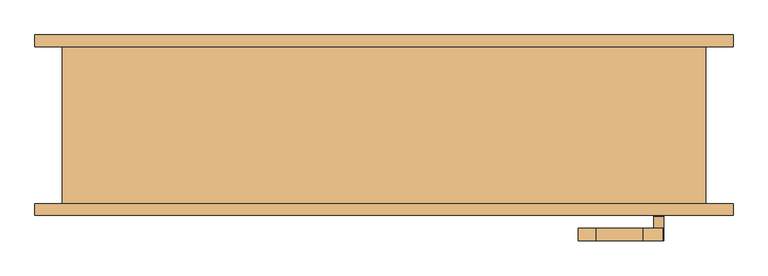
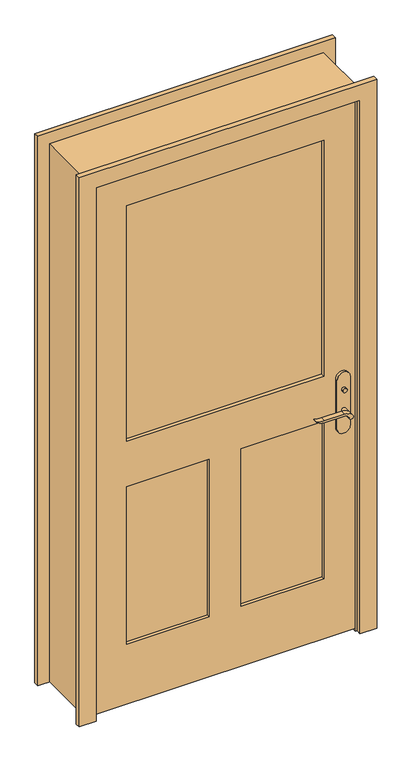
"""IFC4 building model written with IfcOpenShell, lengths in millimetres: door geometry."""

import ifcopenshell
import ifcopenshell.guid

model = None  # the IFC model being written
_history = None  # IfcOwnerHistory: only IFC2X3 demands one
_inside = {}  # id of a spatial element -> (the spatial element, [elements in it])
_under = {}  # id of a project, library or spatial element -> (it, [spatial elements below it])
_declared = {}  # id of a project -> (the project, [libraries it declares])
_typed = {}  # id of a type object -> (the type object, [elements of that type])
_made_of = {}  # id of a material, layer set ... -> (it, [elements and type objects made of it])


def new_model(schema):
    """Start an empty IFC model of exactly this schema.

    Asked for "IFC4X3", IfcOpenShell would pick the latest addendum, in which some entities
    have other attributes; the version numbers below select the first issue.
    IFC2X3 requires an IfcOwnerHistory on every rooted entity: one is made here for all.
    """
    global model, _history
    if schema == "IFC4X3":
        model = ifcopenshell.file(schema_version=(4, 3, 0, 0))
    else:
        model = ifcopenshell.file(schema=schema)
    _inside.clear()
    _under.clear()
    _declared.clear()
    _typed.clear()
    _made_of.clear()
    _history = None
    if model.schema == "IFC2X3":
        org = make("IfcOrganization", Name="unknown")
        user = make(
            "IfcPersonAndOrganization",
            ThePerson=make("IfcPerson", FamilyName="unknown"),
            TheOrganization=org,
        )
        app = make(
            "IfcApplication",
            ApplicationDeveloper=org,
            Version="unknown",
            ApplicationFullName="unknown",
            ApplicationIdentifier="unknown",
        )
        _history = make(
            "IfcOwnerHistory",
            OwningUser=user,
            OwningApplication=app,
            ChangeAction="ADDED",
            CreationDate=0,
        )
    return model


def make(cls, **values):
    """One entity of the class cls with the attributes given. An attribute that is None is left unset."""
    return model.create_entity(
        cls, **{name: value for name, value in values.items() if value is not None}
    )


def rooted(cls, **values):
    """An entity with a GlobalId (a new one), such as an element, a storey or a relation."""
    return make(cls, GlobalId=ifcopenshell.guid.new(), OwnerHistory=_history, **values)


def si_unit(unit_type, name, prefix=None):
    """IfcSIUnit, for example si_unit("LENGTHUNIT", "METRE", prefix="MILLI")."""
    return make("IfcSIUnit", UnitType=unit_type, Prefix=prefix, Name=name)


def assignment(units):
    """IfcUnitAssignment: the units of a project."""
    return None if units is None else make("IfcUnitAssignment", Units=units)


def point(xyz):
    """IfcCartesianPoint."""
    return None if xyz is None else make("IfcCartesianPoint", Coordinates=xyz)


def direction(xyz):
    """IfcDirection."""
    return None if xyz is None else make("IfcDirection", DirectionRatios=xyz)


def frame(location, z_axis=None, x_axis=None):
    """IfcAxis2Placement3D, a coordinate frame: its origin and axes. An axis left out is left unset."""
    return make(
        "IfcAxis2Placement3D",
        Location=point(location),
        Axis=direction(z_axis),
        RefDirection=direction(x_axis),
    )


def frame_2d(location, x_axis=None):
    """IfcAxis2Placement2D, a coordinate frame in the plane: its origin and x axis."""
    return make(
        "IfcAxis2Placement2D", Location=point(location), RefDirection=direction(x_axis)
    )


def origin():
    """The frame at (0, 0, 0) with its axes left unset."""
    return frame((0.0, 0.0, 0.0))


def place(relative_to, where):
    """IfcLocalPlacement: puts the frame where relative to a parent placement (None: the world)."""
    return make(
        "IfcLocalPlacement", PlacementRelTo=relative_to, RelativePlacement=where
    )


def context(
    kind, dimensions, precision=None, world=None, true_north=None, identifier=None
):
    """IfcGeometricRepresentationContext, for example the 3D "Model" context."""
    return make(
        "IfcGeometricRepresentationContext",
        ContextIdentifier=identifier,
        ContextType=kind,
        CoordinateSpaceDimension=dimensions,
        Precision=precision,
        WorldCoordinateSystem=world,
        TrueNorth=true_north,
    )


def project(units=None, contexts=None):
    """IfcProject with its units and contexts."""
    return rooted(
        "IfcProject",
        Name="project",
        RepresentationContexts=contexts,
        UnitsInContext=assignment(units),
    )


def spatial(cls, under=None, at=None, **own):
    """A site, building, storey or space (cls), placed at a placement, below another one or the project."""
    s = rooted(cls, ObjectPlacement=at, **own)
    if under is not None:
        _under.setdefault(under.id(), (under, []))[1].append(s)
    return s


def polyline(points):
    """IfcPolyline through the points."""
    return make("IfcPolyline", Points=[point(p) for p in points])


def circle_curve(where, radius):
    """IfcCircle in the frame where."""
    return make("IfcCircle", Position=where, Radius=radius)


def trimmed(basis, trim1, trim2, sense, master):
    """IfcTrimmedCurve: the piece of a basis curve between two trims."""
    return make(
        "IfcTrimmedCurve",
        BasisCurve=basis,
        Trim1=trim1,
        Trim2=trim2,
        SenseAgreement=sense,
        MasterRepresentation=master,
    )


def segment(curve, same_sense, transition):
    """IfcCompositeCurveSegment."""
    return make(
        "IfcCompositeCurveSegment",
        Transition=transition,
        SameSense=same_sense,
        ParentCurve=curve,
    )


def composite_curve(segments, self_intersect=None):
    """IfcCompositeCurve: segments joined end to end."""
    return make("IfcCompositeCurve", Segments=segments, SelfIntersect=self_intersect)


def outline(outer, holes=None, kind="AREA"):
    """IfcArbitraryClosedProfileDef: a profile drawn as a closed curve; with holes, ...WithVoids."""
    if holes is None:
        return make("IfcArbitraryClosedProfileDef", ProfileType=kind, OuterCurve=outer)
    return make(
        "IfcArbitraryProfileDefWithVoids",
        ProfileType=kind,
        OuterCurve=outer,
        InnerCurves=holes,
    )


def extrude(swept, where, along, depth):
    """IfcExtrudedAreaSolid: the profile swept, set in the frame where, extruded along a direction by depth."""
    return make(
        "IfcExtrudedAreaSolid",
        SweptArea=swept,
        Position=where,
        ExtrudedDirection=direction(along),
        Depth=depth,
    )


def faces_of(points, faces, orient=None, outer=None):
    """IfcFace entities. A face is a list of loops; a loop is a list of indices into points, from 0.

    orient and outer hold one flag for each loop. By default every Orientation is true, the
    first loop of a face is its IfcFaceOuterBound and the others are IfcFaceBound.
    """
    made = []
    for i, loops in enumerate(faces):
        bounds = []
        for j, loop in enumerate(loops):
            is_outer = j == 0 if outer is None else outer[i][j]
            bounds.append(
                make(
                    "IfcFaceOuterBound" if is_outer else "IfcFaceBound",
                    Bound=make("IfcPolyLoop", Polygon=[points[k] for k in loop]),
                    Orientation=True if orient is None else orient[i][j],
                )
            )
        made.append(make("IfcFace", Bounds=bounds))
    return made


def faceted_brep(points, faces, orient=None, outer=None, voids=None):
    """IfcFacetedBrep: a solid bounded by flat faces; with voids (closed shells), ...WithVoids."""
    shared = [point(p) for p in points]
    hull = make("IfcClosedShell", CfsFaces=faces_of(shared, faces, orient, outer))
    if voids is None:
        return make("IfcFacetedBrep", Outer=hull)
    return make(
        "IfcFacetedBrepWithVoids",
        Outer=hull,
        Voids=[
            make(cls, CfsFaces=faces_of(shared, fs, o, b)) for cls, fs, o, b in voids
        ],
    )


def shape(context_of_items, identifier, shape_type, items):
    """IfcShapeRepresentation: the items that make up one representation, for example the "Body"."""
    return make(
        "IfcShapeRepresentation",
        ContextOfItems=context_of_items,
        RepresentationIdentifier=identifier,
        RepresentationType=shape_type,
        Items=items,
    )


def source(mapping_origin, context_of_items, identifier, shape_type, items):
    """IfcRepresentationMap: a shape defined once, which mapped items show again and again."""
    return make(
        "IfcRepresentationMap",
        MappingOrigin=mapping_origin,
        MappedRepresentation=shape(context_of_items, identifier, shape_type, items),
    )


def transform(
    local_origin,
    x_axis=None,
    y_axis=None,
    z_axis=None,
    scale=None,
    scale2=None,
    scale3=None,
    uniform=True,
):
    """IfcCartesianTransformationOperator3D, or its non-uniform kind. x_axis, y_axis, z_axis: its Axis1, 2, 3."""
    if uniform:
        return make(
            "IfcCartesianTransformationOperator3D",
            Axis1=direction(x_axis),
            Axis2=direction(y_axis),
            LocalOrigin=point(local_origin),
            Scale=scale,
            Axis3=direction(z_axis),
        )
    return make(
        "IfcCartesianTransformationOperator3DnonUniform",
        Axis1=direction(x_axis),
        Axis2=direction(y_axis),
        LocalOrigin=point(local_origin),
        Scale=scale,
        Axis3=direction(z_axis),
        Scale2=scale2,
        Scale3=scale3,
    )


def mapped(mapping_source, mapping_target):
    """IfcMappedItem: shows the shape of a source again, moved by a transform."""
    return make(
        "IfcMappedItem", MappingSource=mapping_source, MappingTarget=mapping_target
    )


def made_of(thing, what):
    """Note that an element or type object is made of a material, layer set ...; save() writes the relation."""
    if what is not None:
        _made_of.setdefault(what.id(), (what, []))[1].append(thing)
    return thing


def element(
    cls,
    number,
    at=None,
    inside=None,
    cuts=None,
    type_object=None,
    material=None,
    context=None,
    identifier="Body",
    shape_type=None,
    held_by="IfcProductDefinitionShape",
    body=None,
    shapes=None,
    **own,
):
    """One element of the class cls, such as IfcWall. Its Tag is "e" and its number.

    at: its placement. inside: the storey or other place that contains it. cuts: it is an
    opening in that element (IfcRelVoidsElement). A single representation is given by context,
    identifier, shape_type and body (its items); several are given by shapes. held_by: the class
    of the entity that holds the representations. save() writes the other relations.
    """
    e = rooted(cls, Tag="e%d" % number, ObjectPlacement=at, **own)
    if body is not None:
        shapes = [shape(context, identifier, shape_type, body)]
    if shapes is not None:
        e.Representation = make(held_by, Representations=shapes)
    if inside is not None:
        _inside.setdefault(inside.id(), (inside, []))[1].append(e)
    if cuts is not None:
        rooted(
            "IfcRelVoidsElement", RelatingBuildingElement=cuts, RelatedOpeningElement=e
        )
    if type_object is not None:
        _typed.setdefault(type_object.id(), (type_object, []))[1].append(e)
    return made_of(e, material)


def aggregate(whole, parts):
    """IfcRelAggregates: a whole, such as a stair, and the parts it consists of."""
    return rooted("IfcRelAggregates", RelatingObject=whole, RelatedObjects=parts)


def save(model, path):
    """Write the relations noted so far, then the file.

    IfcRelAggregates (storeys below a building ...), IfcRelContainedInSpatialStructure (elements
    in a storey), IfcRelDefinesByType, IfcRelAssociatesMaterial and IfcRelDeclares: one each for
    every whole, place, type object, material and project.
    """
    for whole, parts in _under.values():
        aggregate(whole, parts)
    for where, things in _inside.values():
        rooted(
            "IfcRelContainedInSpatialStructure",
            RelatedElements=things,
            RelatingStructure=where,
        )
    for kind, things in _typed.values():
        rooted("IfcRelDefinesByType", RelatedObjects=things, RelatingType=kind)
    for what, things in _made_of.values():
        rooted("IfcRelAssociatesMaterial", RelatedObjects=things, RelatingMaterial=what)
    for by, libraries in _declared.values():
        rooted("IfcRelDeclares", RelatingContext=by, RelatedDefinitions=libraries)
    model.write(path)


def door_90a51b68(model_context):
    return source(origin(), model_context, "Body", "SolidModel", [
        extrude(outline(polyline([(-38.1, 12.7), (-12.7, 0.0), (-98.425, 0.0), (-73.025, 12.7), (-38.1, 12.7)])), frame((-495.3, 0.0, 0.0), z_axis=(1.0, 0.0, 0.0), x_axis=(0.0, 1.0, 0.0)), (0.0, 0.0, 1.0), 990.6),
        extrude(outline(polyline([(449.5, -68.9), (449.5, -78.9), (439.5, -78.9), (439.5, -68.9), (449.5, -68.9)])), frame((0.0, 0.0, 981.9), z_axis=(0.0, 0.0, 1.0), x_axis=(1.0, 0.0, 0.0)), (0.0, 0.0, 1.0), 30.0),
        extrude(outline(composite_curve([segment(trimmed(circle_curve(frame_2d((996.9, 444.5)), 8.0), [point((996.9, 436.5))], [point((996.9, 452.5))], False, "CARTESIAN"), True, "CONTINUOUS"), segment(trimmed(circle_curve(frame_2d((996.9, 444.5)), 8.0), [point((996.9, 452.5))], [point((996.9, 436.5))], False, "CARTESIAN"), True, "CONTINUOUS")], self_intersect=False)), frame((0.0, -143.825, 0.0), z_axis=(0.0, 1.0, 0.0), x_axis=(0.0, 0.0, 1.0)), (0.0, 0.0, 1.0), 10.0),
        extrude(outline(composite_curve([segment(trimmed(circle_curve(frame_2d((897.1555521, 420.8324871)), 37.2832219), [point((919.0523287, 451.0081363))], [point((934.4, 419.1325667))], False, "CARTESIAN"), True, "CONTINUOUS"), segment(polyline([(934.4, 419.1325667), (934.4, 342.8564091)]), True, "CONTINUOUS"), segment(trimmed(circle_curve(frame_2d((1017.6850638, 342.9227909)), 83.2850902), [point((934.4, 342.8564091))], [point((939.4, 314.5))], True, "CARTESIAN"), True, "CONTINUOUS"), segment(polyline([(939.4, 314.5), (936.6135558, 314.5)]), True, "CONTINUOUS"), segment(trimmed(circle_curve(frame_2d((986.6709207, 346.4396612)), 59.3791355), [point((936.6135558, 314.5))], [point((927.4, 342.8564091))], False, "CARTESIAN"), True, "CONTINUOUS"), segment(polyline([(927.4, 342.8564091), (927.4, 419.1138099)]), True, "CONTINUOUS"), segment(trimmed(circle_curve(frame_2d((909.2738613, 419.1138099)), 18.1261387), [point((927.4, 419.1138099))], [point((914.4, 436.5))], True, "CARTESIAN"), True, "CONTINUOUS"), segment(trimmed(circle_curve(frame_2d((914.4, 444.5)), 8.0), [point((914.4, 436.5))], [point((919.0523287, 451.0081363))], False, "CARTESIAN"), True, "CONTINUOUS")], self_intersect=False)), frame((0.0, -48.9, 0.0), z_axis=(0.0, 1.0, 0.0), x_axis=(0.0, 0.0, 1.0)), (0.0, 0.0, 1.0), 20.0),
        extrude(outline(composite_curve([segment(trimmed(circle_curve(frame_2d((914.4, 444.5)), 8.0), [point((914.3999903, 436.5))], [point((919.0523287, 451.0081363))], False, "CARTESIAN"), True, "CONTINUOUS"), segment(trimmed(circle_curve(frame_2d((897.1555521, 420.8324871)), 37.2832219), [point((919.0523287, 451.0081363))], [point((934.4, 419.1325667))], False, "CARTESIAN"), True, "CONTINUOUS"), segment(polyline([(934.4, 419.1325667), (934.4, 342.8564091)]), True, "CONTINUOUS"), segment(trimmed(circle_curve(frame_2d((1017.6850638, 342.9227909)), 83.2850902), [point((934.4, 342.8564091))], [point((939.4, 314.5))], True, "CARTESIAN"), True, "CONTINUOUS"), segment(polyline([(939.4, 314.5), (936.6135558, 314.5)]), True, "CONTINUOUS"), segment(trimmed(circle_curve(frame_2d((986.6709207, 346.4396612)), 59.3791355), [point((936.6135558, 314.5))], [point((927.4, 342.8564091))], False, "CARTESIAN"), True, "CONTINUOUS"), segment(polyline([(927.4, 342.8564091), (927.4, 419.1138122)]), True, "CONTINUOUS"), segment(trimmed(circle_curve(frame_2d((909.2738682, 419.1138122)), 18.1261318), [point((927.4, 419.1138122))], [point((914.3999903, 436.5))], True, "CARTESIAN"), True, "CONTINUOUS")], self_intersect=False)), frame((0.0, -183.825, 0.0), z_axis=(0.0, 1.0, 0.0), x_axis=(0.0, 0.0, 1.0)), (0.0, 0.0, 1.0), 20.0),
        extrude(outline(composite_curve([segment(trimmed(circle_curve(frame_2d((914.4, 444.5)), 8.0), [point((914.4, 436.5))], [point((914.4, 452.5))], False, "CARTESIAN"), True, "CONTINUOUS"), segment(trimmed(circle_curve(frame_2d((914.4, 444.5)), 8.0), [point((914.4, 452.5))], [point((914.4, 436.5))], False, "CARTESIAN"), True, "CONTINUOUS")], self_intersect=False)), frame((0.0, -78.9, 0.0), z_axis=(0.0, 1.0, 0.0), x_axis=(0.0, 0.0, 1.0)), (0.0, 0.0, 1.0), 30.0),
        extrude(outline(composite_curve([segment(trimmed(circle_curve(frame_2d((914.4, 444.5)), 8.0), [point((914.4, 436.5))], [point((914.4, 452.5))], False, "CARTESIAN"), True, "CONTINUOUS"), segment(trimmed(circle_curve(frame_2d((914.4, 444.5)), 8.0), [point((914.4, 452.5))], [point((914.4, 436.5))], False, "CARTESIAN"), True, "CONTINUOUS")], self_intersect=False)), frame((0.0, -163.825, 0.0), z_axis=(0.0, 1.0, 0.0), x_axis=(0.0, 0.0, 1.0)), (0.0, 0.0, 1.0), 30.0),
        extrude(outline(composite_curve([segment(polyline([(844.4, 469.5), (1039.4, 469.5)]), True, "CONTINUOUS"), segment(trimmed(circle_curve(frame_2d((1039.4, 444.5)), 25.0), [point((1039.4, 469.5))], [point((1039.4, 419.5))], False, "CARTESIAN"), True, "CONTINUOUS"), segment(polyline([(1039.4, 419.5), (844.4, 419.5)]), True, "CONTINUOUS"), segment(trimmed(circle_curve(frame_2d((844.4, 444.5)), 25.0), [point((844.4, 419.5))], [point((844.4, 469.5))], False, "CARTESIAN"), True, "CONTINUOUS")], self_intersect=False)), frame((0.0, -88.9, 0.0), z_axis=(0.0, 1.0, 0.0), x_axis=(0.0, 0.0, 1.0)), (0.0, 0.0, 1.0), 10.0),
        extrude(outline(composite_curve([segment(polyline([(844.4, 469.5), (1039.4, 469.5)]), True, "CONTINUOUS"), segment(trimmed(circle_curve(frame_2d((1039.4, 444.5)), 25.0), [point((1039.4, 469.5))], [point((1039.4, 419.5))], False, "CARTESIAN"), True, "CONTINUOUS"), segment(polyline([(1039.4, 419.5), (844.4, 419.5)]), True, "CONTINUOUS"), segment(trimmed(circle_curve(frame_2d((844.4, 444.5)), 25.0), [point((844.4, 419.5))], [point((844.4, 469.5))], False, "CARTESIAN"), True, "CONTINUOUS")], self_intersect=False)), frame((0.0, -133.825, 0.0), z_axis=(0.0, 1.0, 0.0), x_axis=(0.0, 0.0, 1.0)), (0.0, 0.0, 1.0), 10.0),
        faceted_brep([(520.7, -123.825, 0.0), (495.3, -123.825, 0.0), (495.3, -88.9, 0.0), (482.6, -88.9, 0.0), (482.6, -53.975, 0.0), (495.3, -53.975, 0.0), (495.3, 130.175, 0.0), (520.7, 130.175, 0.0), (520.7, 130.175, 2159.0), (520.7, -123.825, 2159.0), (495.3, 130.175, 2133.6), (-495.3, 130.175, 2133.6), (-495.3, 130.175, 0.0), (-520.7, 130.175, 0.0), (-520.7, 130.175, 2159.0), (495.3, -53.975, 2133.6), (482.6, -53.975, 2120.9), (-482.6, -53.975, 2120.9), (-482.6, -53.975, 0.0), (-495.3, -53.975, 0.0), (-495.3, -53.975, 2133.6), (482.6, -88.9, 2120.9), (495.3, -88.9, 2133.6), (-495.3, -88.9, 2133.6), (-495.3, -88.9, 0.0), (-482.6, -88.9, 0.0), (-482.6, -88.9, 2120.9), (495.3, -123.825, 2133.6), (-520.7, -123.825, 2159.0), (-520.7, -123.825, 0.0), (-495.3, -123.825, 0.0), (-495.3, -123.825, 2133.6)], [[[0, 1, 2, 3, 4, 5, 6, 7]], [[7, 8, 9, 0]], [[6, 10, 11, 12, 13, 14, 8, 7]], [[5, 15, 10, 6]], [[4, 16, 17, 18, 19, 20, 15, 5]], [[3, 21, 16, 4]], [[2, 22, 23, 24, 25, 26, 21, 3]], [[1, 27, 22, 2]], [[0, 9, 28, 29, 30, 31, 27, 1]], [[8, 14, 28, 9]], [[15, 20, 11, 10]], [[21, 26, 17, 16]], [[27, 31, 23, 22]], [[29, 13, 12, 19, 18, 25, 24, 30]], [[14, 13, 29, 28]], [[20, 19, 12, 11]], [[26, 25, 18, 17]], [[31, 30, 24, 23]]]),
        extrude(outline(polyline([(2133.6, -495.3), (12.7, -495.3), (12.7, 495.3), (2133.6, 495.3), (2133.6, -495.3)]), holes=[polyline([(1066.8, -374.65), (2012.95, -374.65), (2012.95, 374.65), (1066.8, 374.65), (1066.8, -374.65)]), polyline([(885.825, -60.325), (254.0, -60.325), (254.0, -374.65), (885.825, -374.65), (885.825, -60.325)]), polyline([(885.825, 374.65), (254.0, 374.65), (254.0, 60.325), (885.825, 60.325), (885.825, 374.65)])]), frame((0.0, -123.825, 0.0), z_axis=(0.0, 1.0, 0.0), x_axis=(0.0, 0.0, 1.0)), (0.0, 0.0, 1.0), 34.925),
        extrude(outline(polyline([(374.65, -102.87), (374.65, -109.855), (-374.65, -109.855), (-374.65, -102.87), (374.65, -102.87)])), frame((0.0, 0.0, 1066.8), z_axis=(0.0, 0.0, 1.0), x_axis=(1.0, 0.0, 0.0)), (0.0, 0.0, 1.0), 946.15),
        extrude(outline(polyline([(-60.325, -100.5416667), (-60.325, -112.1833333), (-374.65, -112.1833333), (-374.65, -100.5416667), (-60.325, -100.5416667)])), frame((0.0, 0.0, 254.0), z_axis=(0.0, 0.0, 1.0), x_axis=(1.0, 0.0, 0.0)), (0.0, 0.0, 1.0), 631.825),
        extrude(outline(polyline([(374.65, -100.5416667), (374.65, -112.1833333), (60.325, -112.1833333), (60.325, -100.5416667), (374.65, -100.5416667)])), frame((0.0, 0.0, 254.0), z_axis=(0.0, 0.0, 1.0), x_axis=(1.0, 0.0, 0.0)), (0.0, 0.0, 1.0), 631.825),
        extrude(outline(polyline([(0.0, -501.65), (2139.95, -501.65), (2139.95, 501.65), (0.0, 501.65), (0.0, 565.15), (2203.45, 565.15), (2203.45, -565.15), (0.0, -565.15), (0.0, -501.65)])), frame((0.0, -142.875, 0.0), z_axis=(0.0, 1.0, 0.0), x_axis=(0.0, 0.0, 1.0)), (0.0, 0.0, 1.0), 19.05),
        extrude(outline(polyline([(0.0, -501.65), (2139.95, -501.65), (2139.95, 501.65), (0.0, 501.65), (0.0, 565.15), (2203.45, 565.15), (2203.45, -565.15), (0.0, -565.15), (0.0, -501.65)])), frame((0.0, 130.175, 0.0), z_axis=(0.0, 1.0, 0.0), x_axis=(0.0, 0.0, 1.0)), (0.0, 0.0, 1.0), 19.05),
    ])


if __name__ == "__main__":
    model = new_model("IFC4")
    model_context = context("Model", 3, world=origin())
    ifc_project = project(units=[si_unit("LENGTHUNIT", "METRE", prefix="MILLI")], contexts=[model_context])
    site = spatial("IfcSite", under=ifc_project)
    building = spatial("IfcBuilding", under=site)
    placement = place(None, origin())
    door_shape = door_90a51b68(model_context)
    element("IfcDoor", 1, ObjectType="Door-Exterior-Single-Entry-Half Flat Glass-Wood_Clad : 3'3\"*7' Door", at=placement, inside=building, context=model_context, shape_type="MappedRepresentation", body=[
        mapped(door_shape, transform((0.0, 0.0, 0.0), x_axis=(1.0, 0.0, 0.0), y_axis=(0.0, 1.0, 0.0), z_axis=(0.0, 0.0, 1.0))),
    ])
    save(model, "model.ifc")

# Revit data of these elements
# Type "Door-Exterior-Single-Entry-Half Flat Glass-Wood_Clad : 3'3\"*7' Door"
#   Type Mark = "9"
#   Assembly Code = "B2030100"
#   Analytic Construction = "French door, wood frame with single glass"
#   Top Rail = 0' - 4 3/4"
#   Threshold Offset [instance default] = 0' - 0 1/2"
#   Thickness = 0' - 1 3/8"
#   Thermal Resistance (R) = 1.0696 (h·ft²·°F)/BTU
#   Swing Angle [instance default] = 90.00°
#   Stiles = 0' - 4 3/4"
#   Rough Width = 3' - 5"
#   Rough Height = 7' - 1"
#   Lock Rail = 0' - 7 1/8"
#   Height = 7' - 0"
#   Width = 3' - 3"
#   Heat Transfer Coefficient (U) = 0.9350 BTU/(h·ft²·°F)
#   Door Offset [instance default] = 0' - 0"
#   Bottom Rail = 0' - 9 1/2"
#   Threshold [instance default] = yes
#   Function = 1
#   Exterior Trim [instance default] = yes
#   Trim Material = Cherry
#   Threshold Material = Cherry
#   Panel Material = Cherry
#   Glazing = Glass
#   Frame Material = Cherry
#   Door Handle Material = Aluminum
#   Visual Light Transmittance = 0
#   Solar Heat Gain Coefficient = 0
#   Wall Closure = (empty or 0)
#   Construction Type = (empty or 0)
# Element 1 (IfcDoor, "Door-Exterior-Single-Entry-Half Flat Glass-Wood_Clad : 3'3\"*7' Door")
#   Materials on its faces: "Cherry", "Aluminum", "Glass"
# Materials
#   "Cherry": class "Wood", colour RGB 226 177 128, transparency 0, Description = "Prunus Serotina", Cost = 0
#   "Glass": class "Glass", colour RGB 0 128 192, transparency 0.75, Description = "Soda Lime Glass", Cost = 0
#   "Aluminum": class "Metal", colour RGB 247 247 247, transparency 0, Description = "Aluminum 6061", Cost = 0
